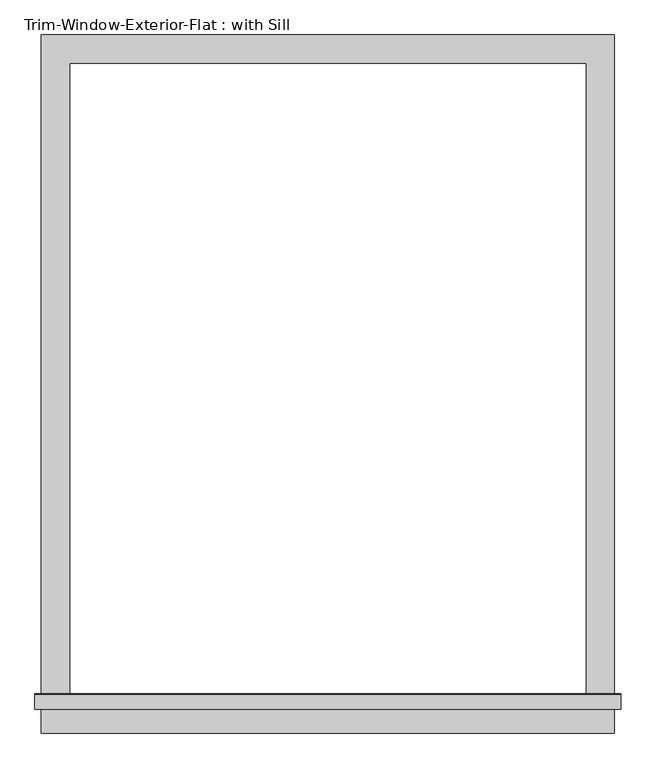
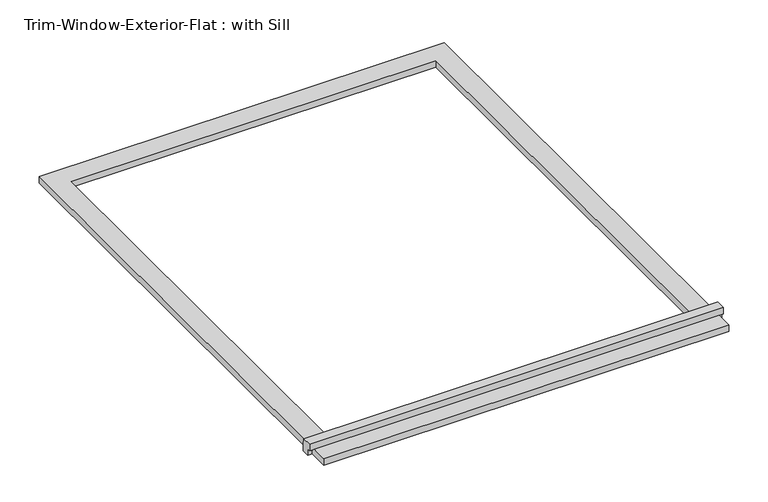
"""IFC4 building model written with IfcOpenShell, lengths in millimetres: proxy geometry, Trim-Window-Exterior-Flat : with Sill."""

import ifcopenshell
import ifcopenshell.guid

model = None  # the IFC model being written
_history = None  # IfcOwnerHistory: only IFC2X3 demands one
_inside = {}  # id of a spatial element -> (the spatial element, [elements in it])
_under = {}  # id of a project, library or spatial element -> (it, [spatial elements below it])
_declared = {}  # id of a project -> (the project, [libraries it declares])
_typed = {}  # id of a type object -> (the type object, [elements of that type])
_made_of = {}  # id of a material, layer set ... -> (it, [elements and type objects made of it])


def new_model(schema):
    """Start an empty IFC model of exactly this schema.

    Asked for "IFC4X3", IfcOpenShell would pick the latest addendum, in which some entities
    have other attributes; the version numbers below select the first issue.
    IFC2X3 requires an IfcOwnerHistory on every rooted entity: one is made here for all.
    """
    global model, _history
    if schema == "IFC4X3":
        model = ifcopenshell.file(schema_version=(4, 3, 0, 0))
    else:
        model = ifcopenshell.file(schema=schema)
    _inside.clear()
    _under.clear()
    _declared.clear()
    _typed.clear()
    _made_of.clear()
    _history = None
    if model.schema == "IFC2X3":
        org = make("IfcOrganization", Name="unknown")
        user = make(
            "IfcPersonAndOrganization",
            ThePerson=make("IfcPerson", FamilyName="unknown"),
            TheOrganization=org,
        )
        app = make(
            "IfcApplication",
            ApplicationDeveloper=org,
            Version="unknown",
            ApplicationFullName="unknown",
            ApplicationIdentifier="unknown",
        )
        _history = make(
            "IfcOwnerHistory",
            OwningUser=user,
            OwningApplication=app,
            ChangeAction="ADDED",
            CreationDate=0,
        )
    return model


def make(cls, **values):
    """One entity of the class cls with the attributes given. An attribute that is None is left unset."""
    return model.create_entity(
        cls, **{name: value for name, value in values.items() if value is not None}
    )


def rooted(cls, **values):
    """An entity with a GlobalId (a new one), such as an element, a storey or a relation."""
    return make(cls, GlobalId=ifcopenshell.guid.new(), OwnerHistory=_history, **values)


def si_unit(unit_type, name, prefix=None):
    """IfcSIUnit, for example si_unit("LENGTHUNIT", "METRE", prefix="MILLI")."""
    return make("IfcSIUnit", UnitType=unit_type, Prefix=prefix, Name=name)


def assignment(units):
    """IfcUnitAssignment: the units of a project."""
    return None if units is None else make("IfcUnitAssignment", Units=units)


def point(xyz):
    """IfcCartesianPoint."""
    return None if xyz is None else make("IfcCartesianPoint", Coordinates=xyz)


def direction(xyz):
    """IfcDirection."""
    return None if xyz is None else make("IfcDirection", DirectionRatios=xyz)


def frame(location, z_axis=None, x_axis=None):
    """IfcAxis2Placement3D, a coordinate frame: its origin and axes. An axis left out is left unset."""
    return make(
        "IfcAxis2Placement3D",
        Location=point(location),
        Axis=direction(z_axis),
        RefDirection=direction(x_axis),
    )


def origin():
    """The frame at (0, 0, 0) with its axes left unset."""
    return frame((0.0, 0.0, 0.0))


def origin_with_axes():
    """The frame at (0, 0, 0) with the z axis (0, 0, 1) and the x axis (1, 0, 0) written out."""
    return frame((0.0, 0.0, 0.0), z_axis=(0.0, 0.0, 1.0), x_axis=(1.0, 0.0, 0.0))


def place(relative_to, where):
    """IfcLocalPlacement: puts the frame where relative to a parent placement (None: the world)."""
    return make(
        "IfcLocalPlacement", PlacementRelTo=relative_to, RelativePlacement=where
    )


def context(
    kind, dimensions, precision=None, world=None, true_north=None, identifier=None
):
    """IfcGeometricRepresentationContext, for example the 3D "Model" context."""
    return make(
        "IfcGeometricRepresentationContext",
        ContextIdentifier=identifier,
        ContextType=kind,
        CoordinateSpaceDimension=dimensions,
        Precision=precision,
        WorldCoordinateSystem=world,
        TrueNorth=true_north,
    )


def project(units=None, contexts=None):
    """IfcProject with its units and contexts."""
    return rooted(
        "IfcProject",
        Name="project",
        RepresentationContexts=contexts,
        UnitsInContext=assignment(units),
    )


def spatial(cls, under=None, at=None, **own):
    """A site, building, storey or space (cls), placed at a placement, below another one or the project."""
    s = rooted(cls, ObjectPlacement=at, **own)
    if under is not None:
        _under.setdefault(under.id(), (under, []))[1].append(s)
    return s


def polyline(points):
    """IfcPolyline through the points."""
    return make("IfcPolyline", Points=[point(p) for p in points])


def outline(outer, holes=None, kind="AREA"):
    """IfcArbitraryClosedProfileDef: a profile drawn as a closed curve; with holes, ...WithVoids."""
    if holes is None:
        return make("IfcArbitraryClosedProfileDef", ProfileType=kind, OuterCurve=outer)
    return make(
        "IfcArbitraryProfileDefWithVoids",
        ProfileType=kind,
        OuterCurve=outer,
        InnerCurves=holes,
    )


def extrude(swept, where, along, depth):
    """IfcExtrudedAreaSolid: the profile swept, set in the frame where, extruded along a direction by depth."""
    return make(
        "IfcExtrudedAreaSolid",
        SweptArea=swept,
        Position=where,
        ExtrudedDirection=direction(along),
        Depth=depth,
    )


def shape(context_of_items, identifier, shape_type, items):
    """IfcShapeRepresentation: the items that make up one representation, for example the "Body"."""
    return make(
        "IfcShapeRepresentation",
        ContextOfItems=context_of_items,
        RepresentationIdentifier=identifier,
        RepresentationType=shape_type,
        Items=items,
    )


def source(mapping_origin, context_of_items, identifier, shape_type, items):
    """IfcRepresentationMap: a shape defined once, which mapped items show again and again."""
    return make(
        "IfcRepresentationMap",
        MappingOrigin=mapping_origin,
        MappedRepresentation=shape(context_of_items, identifier, shape_type, items),
    )


def transform(
    local_origin,
    x_axis=None,
    y_axis=None,
    z_axis=None,
    scale=None,
    scale2=None,
    scale3=None,
    uniform=True,
):
    """IfcCartesianTransformationOperator3D, or its non-uniform kind. x_axis, y_axis, z_axis: its Axis1, 2, 3."""
    if uniform:
        return make(
            "IfcCartesianTransformationOperator3D",
            Axis1=direction(x_axis),
            Axis2=direction(y_axis),
            LocalOrigin=point(local_origin),
            Scale=scale,
            Axis3=direction(z_axis),
        )
    return make(
        "IfcCartesianTransformationOperator3DnonUniform",
        Axis1=direction(x_axis),
        Axis2=direction(y_axis),
        LocalOrigin=point(local_origin),
        Scale=scale,
        Axis3=direction(z_axis),
        Scale2=scale2,
        Scale3=scale3,
    )


def mapped(mapping_source, mapping_target):
    """IfcMappedItem: shows the shape of a source again, moved by a transform."""
    return make(
        "IfcMappedItem", MappingSource=mapping_source, MappingTarget=mapping_target
    )


def made_of(thing, what):
    """Note that an element or type object is made of a material, layer set ...; save() writes the relation."""
    if what is not None:
        _made_of.setdefault(what.id(), (what, []))[1].append(thing)
    return thing


def element(
    cls,
    number,
    at=None,
    inside=None,
    cuts=None,
    type_object=None,
    material=None,
    context=None,
    identifier="Body",
    shape_type=None,
    held_by="IfcProductDefinitionShape",
    body=None,
    shapes=None,
    **own,
):
    """One element of the class cls, such as IfcWall. Its Tag is "e" and its number.

    at: its placement. inside: the storey or other place that contains it. cuts: it is an
    opening in that element (IfcRelVoidsElement). A single representation is given by context,
    identifier, shape_type and body (its items); several are given by shapes. held_by: the class
    of the entity that holds the representations. save() writes the other relations.
    """
    e = rooted(cls, Tag="e%d" % number, ObjectPlacement=at, **own)
    if body is not None:
        shapes = [shape(context, identifier, shape_type, body)]
    if shapes is not None:
        e.Representation = make(held_by, Representations=shapes)
    if inside is not None:
        _inside.setdefault(inside.id(), (inside, []))[1].append(e)
    if cuts is not None:
        rooted(
            "IfcRelVoidsElement", RelatingBuildingElement=cuts, RelatedOpeningElement=e
        )
    if type_object is not None:
        _typed.setdefault(type_object.id(), (type_object, []))[1].append(e)
    return made_of(e, material)


def aggregate(whole, parts):
    """IfcRelAggregates: a whole, such as a stair, and the parts it consists of."""
    return rooted("IfcRelAggregates", RelatingObject=whole, RelatedObjects=parts)


def save(model, path):
    """Write the relations noted so far, then the file.

    IfcRelAggregates (storeys below a building ...), IfcRelContainedInSpatialStructure (elements
    in a storey), IfcRelDefinesByType, IfcRelAssociatesMaterial and IfcRelDeclares: one each for
    every whole, place, type object, material and project.
    """
    for whole, parts in _under.values():
        aggregate(whole, parts)
    for where, things in _inside.values():
        rooted(
            "IfcRelContainedInSpatialStructure",
            RelatedElements=things,
            RelatingStructure=where,
        )
    for kind, things in _typed.values():
        rooted("IfcRelDefinesByType", RelatedObjects=things, RelatingType=kind)
    for what, things in _made_of.values():
        rooted("IfcRelAssociatesMaterial", RelatedObjects=things, RelatingMaterial=what)
    for by, libraries in _declared.values():
        rooted("IfcRelDeclares", RelatingContext=by, RelatedDefinitions=libraries)
    model.write(path)


def trim_window_exterior_flat_with_sill_1cb468f7(model_context):
    return source(origin(), model_context, "Body", "SweptSolid", [
        extrude(outline(polyline([(577.85, -1292.1823709), (577.85, -1349.3323709), (-577.85, -1349.3323709), (-577.85, -1292.1823709), (577.85, -1292.1823709)])), origin_with_axes(), (0.0, 0.0, 1.0), 19.05),
        extrude(outline(polyline([(-1301.75, 38.1), (-1272.4580645, 38.1), (-1270.0, 19.05), (-1270.0, 0.0), (-1292.1823709, 0.0), (-1292.1823709, 19.05), (-1301.75, 19.05), (-1301.75, 38.1)])), frame((-590.55, 0.0, 0.0), z_axis=(1.0, 0.0, 0.0), x_axis=(0.0, 1.0, 0.0)), (0.0, 0.0, 1.0), 1181.1),
        extrude(outline(polyline([(-577.85, 57.15), (577.85, 57.15), (577.85, -1270.0), (520.7, -1270.0), (520.7, 0.0), (-520.7, 0.0), (-520.7, -1270.0), (-577.85, -1270.0), (-577.85, 57.15)])), origin_with_axes(), (0.0, 0.0, 1.0), 19.05),
    ])


if __name__ == "__main__":
    model = new_model("IFC4")
    model_context = context("Model", 3, world=origin())
    ifc_project = project(units=[si_unit("LENGTHUNIT", "METRE", prefix="MILLI")], contexts=[model_context])
    site = spatial("IfcSite", under=ifc_project)
    building = spatial("IfcBuilding", under=site)
    placement = place(None, origin())
    trim_window_exterior_flat_with_sill_shape = trim_window_exterior_flat_with_sill_1cb468f7(model_context)
    element("IfcBuildingElementProxy", 1, Name="Trim-Window-Exterior-Flat : with Sill", ObjectType="Trim-Window-Exterior-Flat : with Sill", at=placement, inside=building, context=model_context, shape_type="MappedRepresentation", body=[
        mapped(trim_window_exterior_flat_with_sill_shape, transform((0.0, 0.0, 0.0), x_axis=(1.0, 0.0, 0.0), y_axis=(0.0, 1.0, 0.0), z_axis=(0.0, 0.0, 1.0))),
    ])
    save(model, "model.ifc")

# Revit data of these elements
# Type "Trim-Window-Exterior-Flat : with Sill"
#   Trim Width = 0' - 2 1/4"
#   Trim Thickness_Picture Frame = 0' - 1 1/4"
#   Trim Thickness_with Sill = 0' - 0 3/4"
#   Sill Thickness = 0' - 1 1/4"
#   Opening Width [instance default] = 2' - 0"
#   Opening Height [instance default] = 3' - 0"
#   Default Elevation = 4' - 0"
#   Sill = yes
#   Picture Frame = no
#   Trim Material [instance default] = none
# Element 1 (IfcBuildingElementProxy, "Trim-Window-Exterior-Flat : with Sill")
#   Opening Width = 3' - 5"
#   Opening Height = 4' - 2"
#   Trim Material = Clad - White
#   Materials on its faces: "Clad - White"
# Materials
#   "Clad - White": class "Wood", colour RGB 242 242 238, transparency 0, Cost = 0
